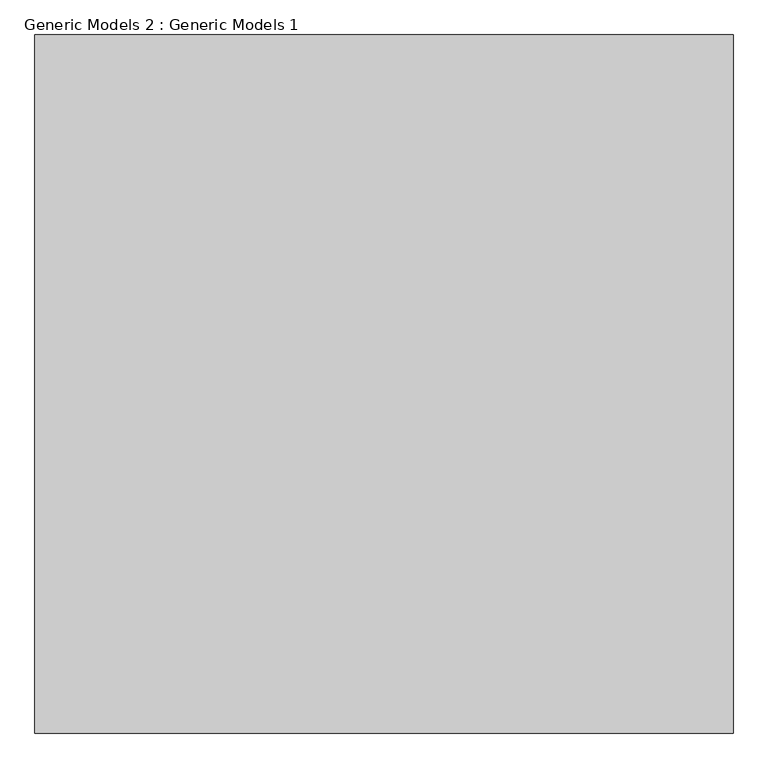
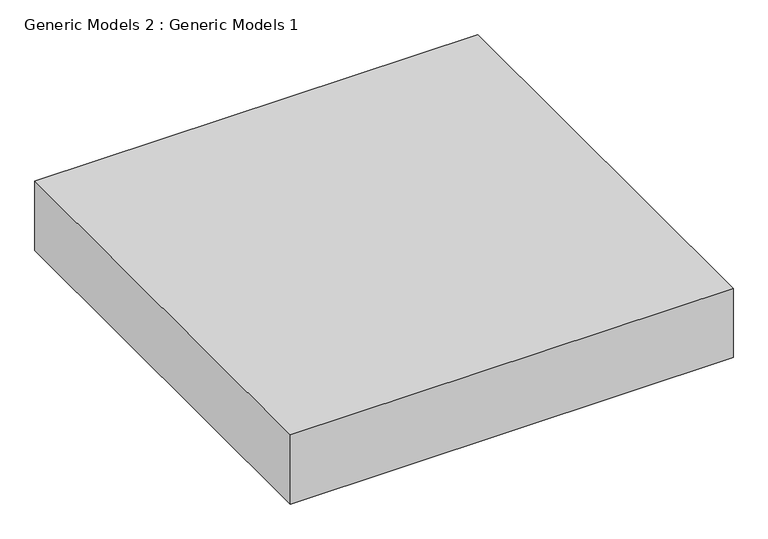
"""IFC4 building model written with IfcOpenShell, lengths in millimetres: proxy geometry, Generic Models 2 : Generic Models 1."""

import ifcopenshell
import ifcopenshell.guid

model = None  # the IFC model being written
_history = None  # IfcOwnerHistory: only IFC2X3 demands one
_inside = {}  # id of a spatial element -> (the spatial element, [elements in it])
_under = {}  # id of a project, library or spatial element -> (it, [spatial elements below it])
_declared = {}  # id of a project -> (the project, [libraries it declares])
_typed = {}  # id of a type object -> (the type object, [elements of that type])
_made_of = {}  # id of a material, layer set ... -> (it, [elements and type objects made of it])


def new_model(schema):
    """Start an empty IFC model of exactly this schema.

    Asked for "IFC4X3", IfcOpenShell would pick the latest addendum, in which some entities
    have other attributes; the version numbers below select the first issue.
    IFC2X3 requires an IfcOwnerHistory on every rooted entity: one is made here for all.
    """
    global model, _history
    if schema == "IFC4X3":
        model = ifcopenshell.file(schema_version=(4, 3, 0, 0))
    else:
        model = ifcopenshell.file(schema=schema)
    _inside.clear()
    _under.clear()
    _declared.clear()
    _typed.clear()
    _made_of.clear()
    _history = None
    if model.schema == "IFC2X3":
        org = make("IfcOrganization", Name="unknown")
        user = make(
            "IfcPersonAndOrganization",
            ThePerson=make("IfcPerson", FamilyName="unknown"),
            TheOrganization=org,
        )
        app = make(
            "IfcApplication",
            ApplicationDeveloper=org,
            Version="unknown",
            ApplicationFullName="unknown",
            ApplicationIdentifier="unknown",
        )
        _history = make(
            "IfcOwnerHistory",
            OwningUser=user,
            OwningApplication=app,
            ChangeAction="ADDED",
            CreationDate=0,
        )
    return model


def make(cls, **values):
    """One entity of the class cls with the attributes given. An attribute that is None is left unset."""
    return model.create_entity(
        cls, **{name: value for name, value in values.items() if value is not None}
    )


def rooted(cls, **values):
    """An entity with a GlobalId (a new one), such as an element, a storey or a relation."""
    return make(cls, GlobalId=ifcopenshell.guid.new(), OwnerHistory=_history, **values)


def si_unit(unit_type, name, prefix=None):
    """IfcSIUnit, for example si_unit("LENGTHUNIT", "METRE", prefix="MILLI")."""
    return make("IfcSIUnit", UnitType=unit_type, Prefix=prefix, Name=name)


def assignment(units):
    """IfcUnitAssignment: the units of a project."""
    return None if units is None else make("IfcUnitAssignment", Units=units)


def point(xyz):
    """IfcCartesianPoint."""
    return None if xyz is None else make("IfcCartesianPoint", Coordinates=xyz)


def direction(xyz):
    """IfcDirection."""
    return None if xyz is None else make("IfcDirection", DirectionRatios=xyz)


def frame(location, z_axis=None, x_axis=None):
    """IfcAxis2Placement3D, a coordinate frame: its origin and axes. An axis left out is left unset."""
    return make(
        "IfcAxis2Placement3D",
        Location=point(location),
        Axis=direction(z_axis),
        RefDirection=direction(x_axis),
    )


def origin():
    """The frame at (0, 0, 0) with its axes left unset."""
    return frame((0.0, 0.0, 0.0))


def origin_with_axes():
    """The frame at (0, 0, 0) with the z axis (0, 0, 1) and the x axis (1, 0, 0) written out."""
    return frame((0.0, 0.0, 0.0), z_axis=(0.0, 0.0, 1.0), x_axis=(1.0, 0.0, 0.0))


def place(relative_to, where):
    """IfcLocalPlacement: puts the frame where relative to a parent placement (None: the world)."""
    return make(
        "IfcLocalPlacement", PlacementRelTo=relative_to, RelativePlacement=where
    )


def context(
    kind, dimensions, precision=None, world=None, true_north=None, identifier=None
):
    """IfcGeometricRepresentationContext, for example the 3D "Model" context."""
    return make(
        "IfcGeometricRepresentationContext",
        ContextIdentifier=identifier,
        ContextType=kind,
        CoordinateSpaceDimension=dimensions,
        Precision=precision,
        WorldCoordinateSystem=world,
        TrueNorth=true_north,
    )


def project(units=None, contexts=None):
    """IfcProject with its units and contexts."""
    return rooted(
        "IfcProject",
        Name="project",
        RepresentationContexts=contexts,
        UnitsInContext=assignment(units),
    )


def spatial(cls, under=None, at=None, **own):
    """A site, building, storey or space (cls), placed at a placement, below another one or the project."""
    s = rooted(cls, ObjectPlacement=at, **own)
    if under is not None:
        _under.setdefault(under.id(), (under, []))[1].append(s)
    return s


def polyline(points):
    """IfcPolyline through the points."""
    return make("IfcPolyline", Points=[point(p) for p in points])


def outline(outer, holes=None, kind="AREA"):
    """IfcArbitraryClosedProfileDef: a profile drawn as a closed curve; with holes, ...WithVoids."""
    if holes is None:
        return make("IfcArbitraryClosedProfileDef", ProfileType=kind, OuterCurve=outer)
    return make(
        "IfcArbitraryProfileDefWithVoids",
        ProfileType=kind,
        OuterCurve=outer,
        InnerCurves=holes,
    )


def extrude(swept, where, along, depth):
    """IfcExtrudedAreaSolid: the profile swept, set in the frame where, extruded along a direction by depth."""
    return make(
        "IfcExtrudedAreaSolid",
        SweptArea=swept,
        Position=where,
        ExtrudedDirection=direction(along),
        Depth=depth,
    )


def shape(context_of_items, identifier, shape_type, items):
    """IfcShapeRepresentation: the items that make up one representation, for example the "Body"."""
    return make(
        "IfcShapeRepresentation",
        ContextOfItems=context_of_items,
        RepresentationIdentifier=identifier,
        RepresentationType=shape_type,
        Items=items,
    )


def source(mapping_origin, context_of_items, identifier, shape_type, items):
    """IfcRepresentationMap: a shape defined once, which mapped items show again and again."""
    return make(
        "IfcRepresentationMap",
        MappingOrigin=mapping_origin,
        MappedRepresentation=shape(context_of_items, identifier, shape_type, items),
    )


def transform(
    local_origin,
    x_axis=None,
    y_axis=None,
    z_axis=None,
    scale=None,
    scale2=None,
    scale3=None,
    uniform=True,
):
    """IfcCartesianTransformationOperator3D, or its non-uniform kind. x_axis, y_axis, z_axis: its Axis1, 2, 3."""
    if uniform:
        return make(
            "IfcCartesianTransformationOperator3D",
            Axis1=direction(x_axis),
            Axis2=direction(y_axis),
            LocalOrigin=point(local_origin),
            Scale=scale,
            Axis3=direction(z_axis),
        )
    return make(
        "IfcCartesianTransformationOperator3DnonUniform",
        Axis1=direction(x_axis),
        Axis2=direction(y_axis),
        LocalOrigin=point(local_origin),
        Scale=scale,
        Axis3=direction(z_axis),
        Scale2=scale2,
        Scale3=scale3,
    )


def mapped(mapping_source, mapping_target):
    """IfcMappedItem: shows the shape of a source again, moved by a transform."""
    return make(
        "IfcMappedItem", MappingSource=mapping_source, MappingTarget=mapping_target
    )


def made_of(thing, what):
    """Note that an element or type object is made of a material, layer set ...; save() writes the relation."""
    if what is not None:
        _made_of.setdefault(what.id(), (what, []))[1].append(thing)
    return thing


def element(
    cls,
    number,
    at=None,
    inside=None,
    cuts=None,
    type_object=None,
    material=None,
    context=None,
    identifier="Body",
    shape_type=None,
    held_by="IfcProductDefinitionShape",
    body=None,
    shapes=None,
    **own,
):
    """One element of the class cls, such as IfcWall. Its Tag is "e" and its number.

    at: its placement. inside: the storey or other place that contains it. cuts: it is an
    opening in that element (IfcRelVoidsElement). A single representation is given by context,
    identifier, shape_type and body (its items); several are given by shapes. held_by: the class
    of the entity that holds the representations. save() writes the other relations.
    """
    e = rooted(cls, Tag="e%d" % number, ObjectPlacement=at, **own)
    if body is not None:
        shapes = [shape(context, identifier, shape_type, body)]
    if shapes is not None:
        e.Representation = make(held_by, Representations=shapes)
    if inside is not None:
        _inside.setdefault(inside.id(), (inside, []))[1].append(e)
    if cuts is not None:
        rooted(
            "IfcRelVoidsElement", RelatingBuildingElement=cuts, RelatedOpeningElement=e
        )
    if type_object is not None:
        _typed.setdefault(type_object.id(), (type_object, []))[1].append(e)
    return made_of(e, material)


def aggregate(whole, parts):
    """IfcRelAggregates: a whole, such as a stair, and the parts it consists of."""
    return rooted("IfcRelAggregates", RelatingObject=whole, RelatedObjects=parts)


def save(model, path):
    """Write the relations noted so far, then the file.

    IfcRelAggregates (storeys below a building ...), IfcRelContainedInSpatialStructure (elements
    in a storey), IfcRelDefinesByType, IfcRelAssociatesMaterial and IfcRelDeclares: one each for
    every whole, place, type object, material and project.
    """
    for whole, parts in _under.values():
        aggregate(whole, parts)
    for where, things in _inside.values():
        rooted(
            "IfcRelContainedInSpatialStructure",
            RelatedElements=things,
            RelatingStructure=where,
        )
    for kind, things in _typed.values():
        rooted("IfcRelDefinesByType", RelatedObjects=things, RelatingType=kind)
    for what, things in _made_of.values():
        rooted("IfcRelAssociatesMaterial", RelatedObjects=things, RelatingMaterial=what)
    for by, libraries in _declared.values():
        rooted("IfcRelDeclares", RelatingContext=by, RelatedDefinitions=libraries)
    model.write(path)


def generic_models_2_generic_models_1_e905d6e5(model_context):
    return source(origin(), model_context, "Body", "SweptSolid", [
        extrude(outline(polyline([(1524.0, 0.0), (0.0, 0.0), (0.0, 1524.0), (1524.0, 1524.0), (1524.0, 0.0)])), origin_with_axes(), (0.0, 0.0, 1.0), 251.7092939),
    ])


if __name__ == "__main__":
    model = new_model("IFC4")
    model_context = context("Model", 3, world=origin())
    ifc_project = project(units=[si_unit("LENGTHUNIT", "METRE", prefix="MILLI")], contexts=[model_context])
    site = spatial("IfcSite", under=ifc_project)
    building = spatial("IfcBuilding", under=site)
    placement = place(None, origin())
    generic_models_2_generic_models_1_shape = generic_models_2_generic_models_1_e905d6e5(model_context)
    element("IfcBuildingElementProxy", 1, Name="Generic Models 2 : Generic Models 1", ObjectType="Generic Models 2 : Generic Models 1", at=placement, inside=building, context=model_context, shape_type="MappedRepresentation", body=[
        mapped(generic_models_2_generic_models_1_shape, transform((0.0, 0.0, 0.0), x_axis=(1.0, 0.0, 0.0), y_axis=(0.0, 1.0, 0.0), z_axis=(0.0, 0.0, 1.0))),
    ])
    save(model, "model.ifc")
